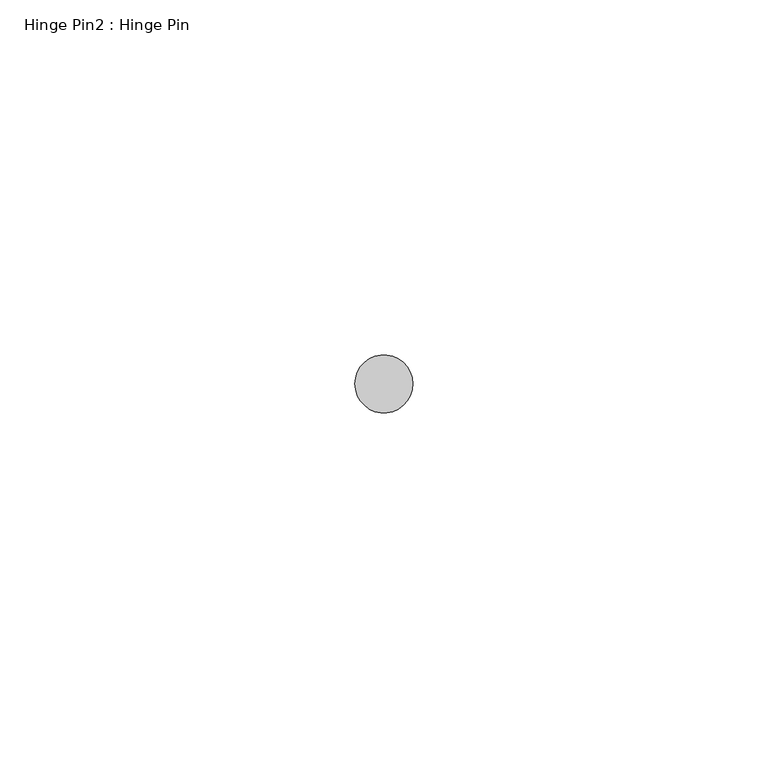
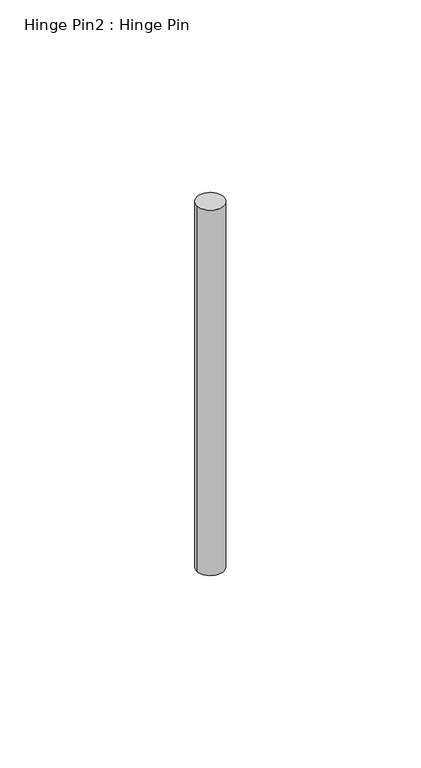
"""IFC4 building model written with IfcOpenShell, lengths in millimetres: proxy geometry, Hinge Pin2 : Hinge Pin."""

from ifc_helpers import new_model, si_unit, point, frame, frame_2d, origin, place, context, project, spatial, circle_curve, trimmed, segment, composite_curve, outline, extrude, source, transform, mapped, element, save


def hinge_pin2_hinge_pin_38e29aa4(model_context):
    return source(origin(), model_context, "Body", "SweptSolid", [
        extrude(outline(composite_curve([segment(trimmed(circle_curve(frame_2d((587319.1320739, -533984.6777841)), 4.0894), [point((587315.0426739, -533984.6777841))], [point((587323.2214739, -533984.6777841))], False, "CARTESIAN"), True, "CONTINUOUS"), segment(trimmed(circle_curve(frame_2d((587319.1320739, -533984.6777841)), 4.0894), [point((587323.2214739, -533984.6777841))], [point((587315.0426739, -533984.6777841))], False, "CARTESIAN"), True, "CONTINUOUS")], self_intersect=False)), frame((0.0, 0.0, 315.7140625), z_axis=(0.0, 0.0, 1.0), x_axis=(1.0, 0.0, 0.0)), (0.0, 0.0, 1.0), 117.871875),
    ])


if __name__ == "__main__":
    model = new_model("IFC4")
    model_context = context("Model", 3, world=origin())
    ifc_project = project(units=[si_unit("LENGTHUNIT", "METRE", prefix="MILLI")], contexts=[model_context])
    site = spatial("IfcSite", under=ifc_project)
    building = spatial("IfcBuilding", under=site)
    placement = place(None, origin())
    hinge_pin2_hinge_pin_shape = hinge_pin2_hinge_pin_38e29aa4(model_context)
    element("IfcBuildingElementProxy", 1, Name="Hinge Pin2 : Hinge Pin", ObjectType="Hinge Pin2 : Hinge Pin", at=placement, inside=building, context=model_context, shape_type="MappedRepresentation", body=[
        mapped(hinge_pin2_hinge_pin_shape, transform((0.0, 0.0, 0.0), x_axis=(1.0, 0.0, 0.0), y_axis=(0.0, 1.0, 0.0), z_axis=(0.0, 0.0, 1.0))),
    ])
    save(model, "model.ifc")

# Revit data of these elements
# Element 1 (IfcBuildingElementProxy, "Hinge Pin2 : Hinge Pin")
#   Materials on its faces: "6\"X6\" WELD-ON STL BUTT HINGE"
# Materials
#   "6\"X6\" WELD-ON STL BUTT HINGE": class "Metal", colour RGB 189 187 185, transparency 0, Description = "Carbon steel", Cost = 0
